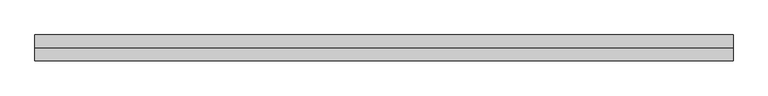
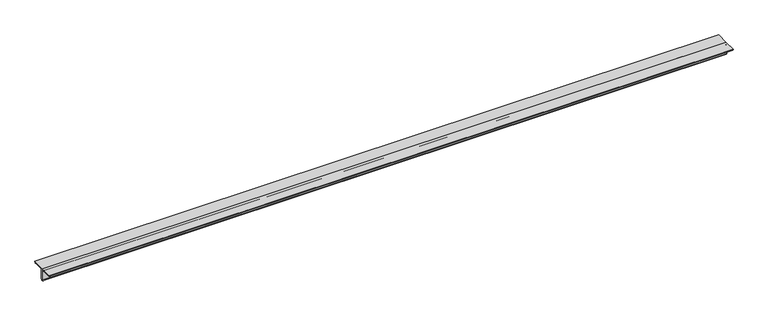
"""IFC4 building model written with IfcOpenShell, lengths in millimetres: member geometry, Steel Framing_2Ls_KS : H_SB_AR_S02_2Ls-100x100x10_VBR1."""

from ifc_helpers import new_model, si_unit, point, frame, frame_2d, origin, place, context, project, spatial, polyline, circle_curve, trimmed, segment, composite_curve, outline, extrude, source, transform, mapped, element, save


def member_a03478a5(model_context):
    return source(origin(), model_context, "Body", "SweptSolid", [
        extrude(outline(composite_curve([segment(polyline([(0.0, 28.2), (100.0, 28.2)]), True, "CONTINUOUS"), segment(trimmed(circle_curve(frame_2d((90.0, 28.2)), 10.0), [point((100.0, 28.2))], [point((90.0, 18.2))], False, "CARTESIAN"), True, "CONTINUOUS"), segment(polyline([(90.0, 18.2), (20.0, 18.2)]), True, "CONTINUOUS"), segment(trimmed(circle_curve(frame_2d((20.0, 8.2)), 10.0), [point((20.0, 18.2))], [point((10.0, 8.2))], True, "CARTESIAN"), True, "CONTINUOUS"), segment(polyline([(10.0, 8.2), (10.0, -61.8)]), True, "CONTINUOUS"), segment(trimmed(circle_curve(frame_2d((0.0, -61.8)), 10.0), [point((10.0, -61.8))], [point((0.0, -71.8))], False, "CARTESIAN"), True, "CONTINUOUS"), segment(polyline([(0.0, -71.8), (0.0, 28.2)]), True, "CONTINUOUS")], self_intersect=False)), frame((-2590.3354834, 0.0, 0.0), z_axis=(1.0, 0.0, 0.0), x_axis=(0.0, 1.0, 0.0)), (0.0, 0.0, 1.0), 5428.7994614),
        extrude(outline(composite_curve([segment(polyline([(0.0, 28.2), (0.0, -71.8)]), True, "CONTINUOUS"), segment(trimmed(circle_curve(frame_2d((0.0, -61.8)), 10.0), [point((0.0, -71.8))], [point((-10.0, -61.8))], False, "CARTESIAN"), True, "CONTINUOUS"), segment(polyline([(-10.0, -61.8), (-10.0, 8.2)]), True, "CONTINUOUS"), segment(trimmed(circle_curve(frame_2d((-20.0, 8.2)), 10.0), [point((-10.0, 8.2))], [point((-20.0, 18.2))], True, "CARTESIAN"), True, "CONTINUOUS"), segment(polyline([(-20.0, 18.2), (-90.0, 18.2)]), True, "CONTINUOUS"), segment(trimmed(circle_curve(frame_2d((-90.0, 28.2)), 10.0), [point((-90.0, 18.2))], [point((-100.0, 28.2))], False, "CARTESIAN"), True, "CONTINUOUS"), segment(polyline([(-100.0, 28.2), (0.0, 28.2)]), True, "CONTINUOUS")], self_intersect=False)), frame((-2590.3354834, 0.0, 0.0), z_axis=(1.0, 0.0, 0.0), x_axis=(0.0, 1.0, 0.0)), (0.0, 0.0, 1.0), 5428.7994614),
    ])


if __name__ == "__main__":
    model = new_model("IFC4")
    model_context = context("Model", 3, world=origin())
    ifc_project = project(units=[si_unit("LENGTHUNIT", "METRE", prefix="MILLI")], contexts=[model_context])
    site = spatial("IfcSite", under=ifc_project)
    building = spatial("IfcBuilding", under=site)
    placement = place(None, origin())
    member_shape = member_a03478a5(model_context)
    element("IfcMember", 1, ObjectType="Steel Framing_2Ls_KS : H_SB_AR_S02_2Ls-100x100x10_VBR1", at=placement, inside=building, context=model_context, shape_type="MappedRepresentation", body=[
        mapped(member_shape, transform((0.0, 0.0, 0.0), x_axis=(1.0, 0.0, 0.0), y_axis=(0.0, 1.0, 0.0), z_axis=(0.0, 0.0, 1.0))),
    ])
    save(model, "model.ifc")

# Revit data of these elements
# Type "Steel Framing_2Ls_KS : H_SB_AR_S02_2Ls-100x100x10_VBR1"
#   Type Comments = "MAIN"
#   Type Mark = "VBR1"
#   H_SectionID = "2Ls-100x100x10"
#   Assembly Code = "B10"
#   Legs = "LLBB"
#   H_Ratio for Additional Steel Plate = 0.2
#   W = 0
#   Perimeter = 0.80 m²/m
#   Nominal Weight = 29.80 kgf/m
#   Length [instance default] = 1524 mm
#   Space = 0 mm
#   b = 100 mm
#   d = 100 mm
#   t = 10 mm
#   y = 28.2 mm
#   A = 0.0038 m²
#   Structural Material [instance default] = Steel, 45-345
# Element 1 (IfcMember, "Steel Framing_2Ls_KS : H_SB_AR_S02_2Ls-100x100x10_VBR1")
#   Materials on its faces: "Steel, 45-345"
# Materials
#   "Steel, 45-345": class "Metal", colour RGB 189 187 185, transparency 0, Description = "Steel 345 MPa", Cost = 0
